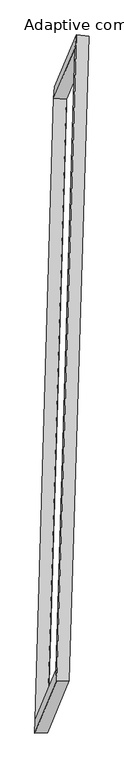
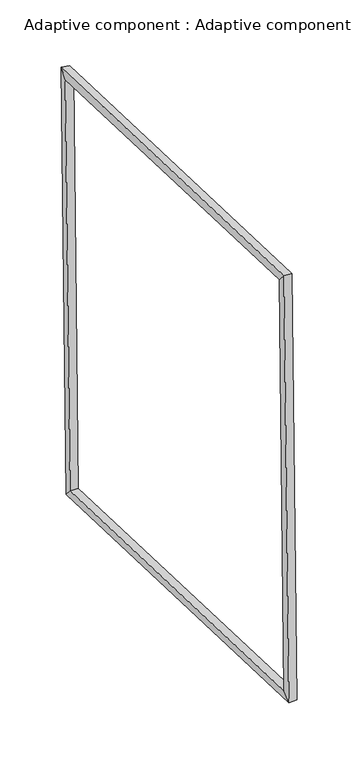
"""IFC4 building model written with IfcOpenShell, lengths in millimetres: proxy geometry, Adaptive component : Adaptive component."""

from ifc_helpers import new_model, si_unit, origin, place, context, project, spatial, faceted_brep, source, transform, mapped, element, save


def adaptive_component_adaptive_component_59bdf4be(model_context):
    return source(origin(), model_context, "Body", "Brep", [
        faceted_brep([(79.8438177, 1311.6078416, 2903.0351871), (144.4746367, 1305.8018165, 2897.9473729), (46.8721959, -1891.3025444, 3146.0959552), (-17.9670892, -1892.3251197, 3151.7137827), (87.3378426, 1381.137173, 2962.5983732), (-14.4225245, -1952.1658792, 3221.3182439), (151.9686616, 1375.3311479, 2957.510559), (50.4167606, -1951.1433039, 3215.7004165), (-61.8727798, -2148.4047439, -209.1371495), (-126.9333874, -2149.9505848, -210.3480384), (-127.5818506, -2219.7047834, -270.115862), (-62.521243, -2218.1589424, -268.9049731), (35.7296609, 1048.699617, -457.2857319), (-29.1224805, 1053.9823765, -459.0266339), (-25.8214835, 1113.5982688, -528.8357327), (39.030658, 1108.3155093, -527.0948306)], [[[0, 1, 2, 3]], [[4, 0, 3, 5]], [[6, 4, 5, 7]], [[1, 6, 7, 2]], [[3, 2, 8, 9]], [[5, 3, 9, 10]], [[7, 5, 10, 11]], [[2, 7, 11, 8]], [[9, 8, 12, 13]], [[10, 9, 13, 14]], [[11, 10, 14, 15]], [[8, 11, 15, 12]], [[13, 12, 1, 0]], [[14, 13, 0, 4]], [[15, 14, 4, 6]], [[12, 15, 6, 1]]]),
    ])


if __name__ == "__main__":
    model = new_model("IFC4")
    model_context = context("Model", 3, world=origin())
    ifc_project = project(units=[si_unit("LENGTHUNIT", "METRE", prefix="MILLI")], contexts=[model_context])
    site = spatial("IfcSite", under=ifc_project)
    building = spatial("IfcBuilding", under=site)
    placement = place(None, origin())
    adaptive_component_adaptive_component_shape = adaptive_component_adaptive_component_59bdf4be(model_context)
    element("IfcBuildingElementProxy", 1, Name="Adaptive component : Adaptive component", ObjectType="Adaptive component : Adaptive component", at=placement, inside=building, context=model_context, shape_type="MappedRepresentation", body=[
        mapped(adaptive_component_adaptive_component_shape, transform((0.0, 0.0, 0.0), x_axis=(1.0, 0.0, 0.0), y_axis=(0.0, 1.0, 0.0), z_axis=(0.0, 0.0, 1.0))),
    ])
    save(model, "model.ifc")

# Revit data of these elements
# Type "Adaptive component : Adaptive component"
#   r [instance default] = 2063.125 mm
#   2r [instance default] = 4126.251 mm
#   Number [instance default] = 5
#   Default Elevation = 0
# Element 1 (IfcBuildingElementProxy, "Adaptive component : Adaptive component")
#   r = 2419.443 mm
#   2r = 4838.886 mm
#   Number = 18
